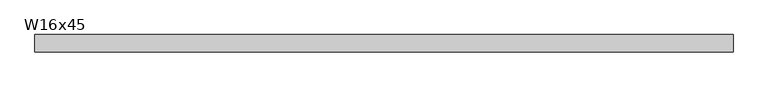
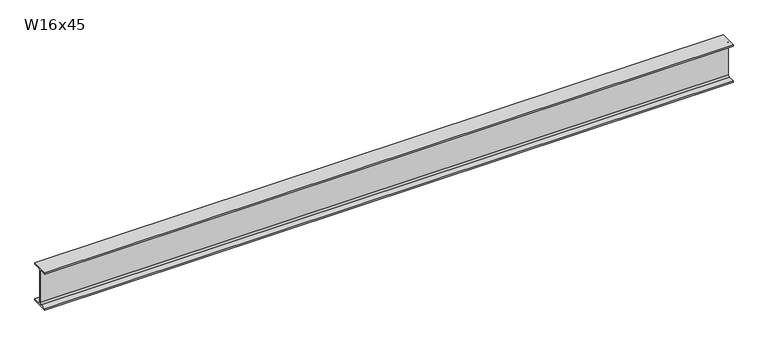
"""IFC4 building model written with IfcOpenShell, lengths in millimetres: beam geometry, RME W-Wide Flange : W16x45."""

from ifc_helpers import new_model, si_unit, point, frame, frame_2d, origin, place, context, project, spatial, polyline, circle_curve, trimmed, segment, composite_curve, outline, extrude, source, transform, mapped, element, save


def w16x45_54da80da(model_context):
    return source(origin(), model_context, "Body", "SweptSolid", [
        extrude(outline(composite_curve([segment(polyline([(89.408, -190.119), (89.408, -204.47), (-89.408, -204.47), (-89.408, -190.119), (-21.7805, -190.119)]), True, "CONTINUOUS"), segment(trimmed(circle_curve(frame_2d((-21.7805, -172.72)), 17.399), [point((-21.7805, -190.119))], [point((-4.3815, -172.72))], True, "CARTESIAN"), True, "CONTINUOUS"), segment(polyline([(-4.3815, -172.72), (-4.3815, 172.72)]), True, "CONTINUOUS"), segment(trimmed(circle_curve(frame_2d((-21.7805, 172.72)), 17.399), [point((-4.3815, 172.72))], [point((-21.7805, 190.119))], True, "CARTESIAN"), True, "CONTINUOUS"), segment(polyline([(-21.7805, 190.119), (-89.408, 190.119), (-89.408, 204.47), (89.408, 204.47), (89.408, 190.119), (21.7805, 190.119)]), True, "CONTINUOUS"), segment(trimmed(circle_curve(frame_2d((21.7805, 172.72)), 17.399), [point((21.7805, 190.119))], [point((4.3815, 172.72))], True, "CARTESIAN"), True, "CONTINUOUS"), segment(polyline([(4.3815, 172.72), (4.3815, -172.72)]), True, "CONTINUOUS"), segment(trimmed(circle_curve(frame_2d((21.7805, -172.72)), 17.399), [point((4.3815, -172.72))], [point((21.7805, -190.119))], True, "CARTESIAN"), True, "CONTINUOUS"), segment(polyline([(21.7805, -190.119), (89.408, -190.119)]), True, "CONTINUOUS")], self_intersect=False)), frame((-3562.7099528, 0.0, 0.0), z_axis=(1.0, 0.0, 0.0), x_axis=(0.0, 1.0, 0.0)), (0.0, 0.0, 1.0), 7135.194165),
    ])


if __name__ == "__main__":
    model = new_model("IFC4")
    model_context = context("Model", 3, world=origin())
    ifc_project = project(units=[si_unit("LENGTHUNIT", "METRE", prefix="MILLI")], contexts=[model_context])
    site = spatial("IfcSite", under=ifc_project)
    building = spatial("IfcBuilding", under=site)
    placement = place(None, origin())
    w16x45_shape = w16x45_54da80da(model_context)
    element("IfcBeam", 1, ObjectType="RME W-Wide Flange : W16x45", at=placement, inside=building, context=model_context, shape_type="MappedRepresentation", body=[
        mapped(w16x45_shape, transform((0.0, 0.0, 0.0), x_axis=(1.0, 0.0, 0.0), y_axis=(0.0, 1.0, 0.0), z_axis=(0.0, 0.0, 1.0))),
    ])
    save(model, "model.ifc")

# Revit data of these elements
# Type "RME W-Wide Flange : W16x45"
#   WELD P [instance default] = ""
#   WELD LE [instance default] = ""
#   WELD D [instance default] = ""
#   TOP SECTION SIZE [instance default] = ""
#   TOP SECTION LENGTH [instance default] = ""
#   REMARKS [instance default] = ""
#   REINF TYPE [instance default] = ""
#   Nominal Size = "W24"
#   End Bearing Capacity [instance default] = ""
#   BOT SECTION SIZE [instance default] = ""
#   BOT SECTION LENGTH [instance default] = ""
#   Assembly Code = "B10"
#   W = 45
#   Start Extension Calculation [instance default] = 10' - 0"
#   Start Extension [instance default] = -0' - 0 1/2"
#   End Extension Calculation [instance default] = 10' - 0"
#   End Extension [instance default] = -0' - 0 1/2"
#   Length [instance default] = 5' - 0"
#   bf = 0' - 7.04"
#   d = 1' - 4.1"
#   k = 0' - 1 1/4"
#   k2 = 0' - 0.685"
#   tf = 0' - 0.565"
#   tw = 0' - 0.345"
#   A = 0.0923611 SF
#   Structural Material [instance default] = Metal - Steel - ASTM A992
# Element 1 (IfcBeam, "RME W-Wide Flange : W16x45")
#   Start Extension Calculation = 9' - 6.39213"
#   Start Extension = -0' - 6.10787"
#   End Extension Calculation = 12' - 1.00046"
#   End Extension = 2' - 0.50046"
#   Length = 24' - 3.74407"
#   Materials on its faces: "Metal - Steel - ASTM A992"
# Materials
#   "Metal - Steel - ASTM A992": class "Metal", colour RGB 255 128 0, transparency 0
